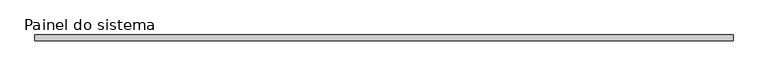
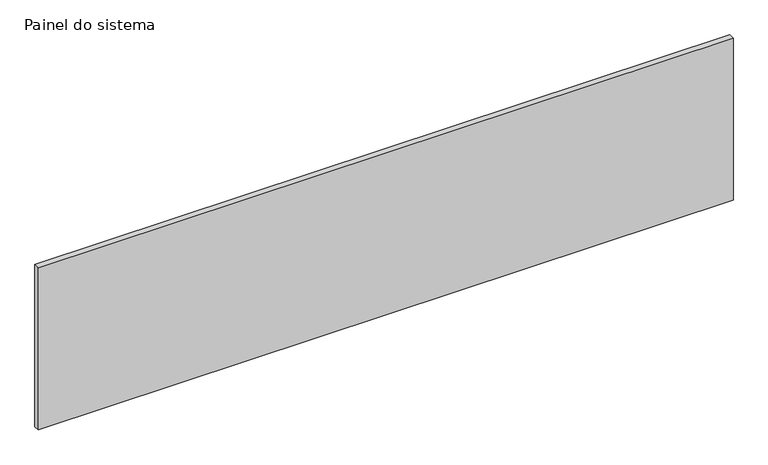
"""IFC4 building model written with IfcOpenShell, lengths in millimetres: plate geometry, Painel do sistema : Envidraçado."""

from ifc_helpers import new_model, si_unit, origin, origin_with_axes, place, context, project, spatial, polyline, outline, extrude, source, transform, mapped, element, save


def painel_do_sistema_bf426e09(model_context):
    return source(origin(), model_context, "Body", "SweptSolid", [
        extrude(outline(polyline([(1475.0, 24.5), (-1475.0, 24.5), (-1475.0, 49.5), (1475.0, 49.5), (1475.0, 24.5)])), origin_with_axes(), (0.0, 0.0, 1.0), 727.4383788),
    ])


if __name__ == "__main__":
    model = new_model("IFC4")
    model_context = context("Model", 3, world=origin())
    ifc_project = project(units=[si_unit("LENGTHUNIT", "METRE", prefix="MILLI")], contexts=[model_context])
    site = spatial("IfcSite", under=ifc_project)
    building = spatial("IfcBuilding", under=site)
    placement = place(None, origin())
    painel_do_sistema_shape = painel_do_sistema_bf426e09(model_context)
    element("IfcPlate", 1, ObjectType="Painel do sistema : Envidraçado", at=placement, inside=building, context=model_context, shape_type="MappedRepresentation", body=[
        mapped(painel_do_sistema_shape, transform((0.0, 0.0, 0.0), x_axis=(1.0, 0.0, 0.0), y_axis=(0.0, 1.0, 0.0), z_axis=(0.0, 0.0, 1.0))),
    ])
    save(model, "model.ifc")

# Revit data of these elements
# Type "Painel do sistema : Envidraçado"
#   Construction Type Id = "GSP4R"
#   Analytic Construction = "Vidraça única Pilkington 1/8 pol"
#   Visual Light Transmittance = 0.9
#   Solar Heat Gain Coefficient = 0.86
#   Heat Transfer Coefficient (U) = 6.7069 W/(m²·K)
# Element 1 (IfcPlate, "Painel do sistema : Envidraçado")
#   Materials on its faces: "Vidro"
# Materials
#   "Vidro": class "Vidro", colour RGB 0 128 192, transparency 0.9, Description = "Vidro de sílica", Cost = 0
